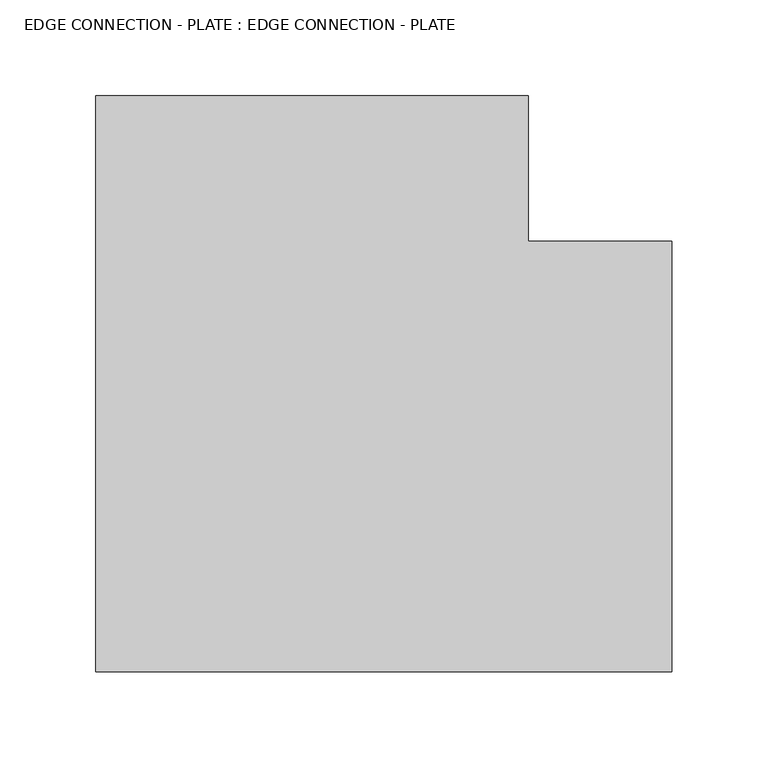
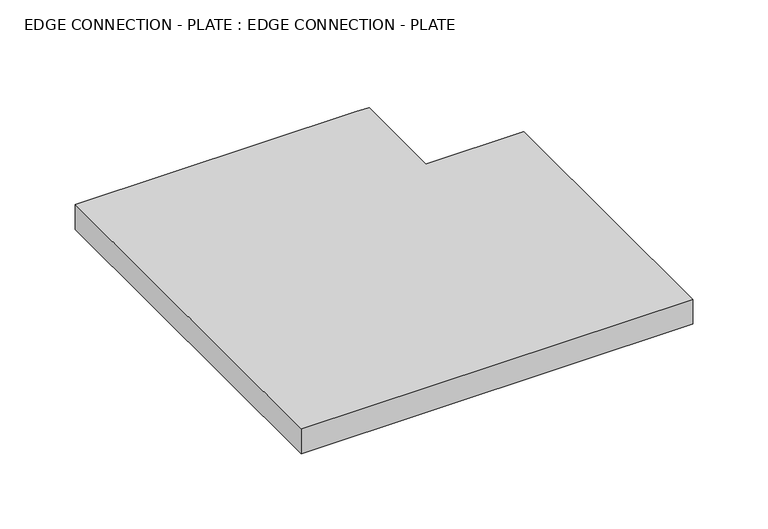
"""IFC4 building model written with IfcOpenShell, lengths in millimetres: fastener geometry, EDGE CONNECTION - PLATE : EDGE CONNECTION - PLATE."""

from ifc_helpers import new_model, si_unit, frame, origin, place, context, project, spatial, polyline, outline, extrude, source, transform, mapped, element, save


def edge_connection_plate_edge_connection_plate_028b5c1e(model_context):
    return source(origin(), model_context, "Body", "SweptSolid", [
        extrude(outline(polyline([(300.0, 19499.5208589), (0.0, 19499.5208589), (0.0, 19799.5208589), (215.138, 19799.5208589), (225.138, 19799.5208589), (225.138, 19723.9908589), (300.0, 19723.9908589), (300.0, 19713.9908589), (300.0, 19499.5208589)])), frame((0.0, 0.0, 330.0), z_axis=(0.0, 0.0, 1.0), x_axis=(1.0, 0.0, 0.0)), (0.0, 0.0, 1.0), 20.0),
    ])


if __name__ == "__main__":
    model = new_model("IFC4")
    model_context = context("Model", 3, world=origin())
    ifc_project = project(units=[si_unit("LENGTHUNIT", "METRE", prefix="MILLI")], contexts=[model_context])
    site = spatial("IfcSite", under=ifc_project)
    building = spatial("IfcBuilding", under=site)
    placement = place(None, origin())
    edge_connection_plate_edge_connection_plate_shape = edge_connection_plate_edge_connection_plate_028b5c1e(model_context)
    element("IfcFastener", 1, ObjectType="EDGE CONNECTION - PLATE : EDGE CONNECTION - PLATE", at=placement, inside=building, context=model_context, shape_type="MappedRepresentation", body=[
        mapped(edge_connection_plate_edge_connection_plate_shape, transform((0.0, 0.0, 0.0), x_axis=(1.0, 0.0, 0.0), y_axis=(0.0, 1.0, 0.0), z_axis=(0.0, 0.0, 1.0))),
    ])
    save(model, "model.ifc")
